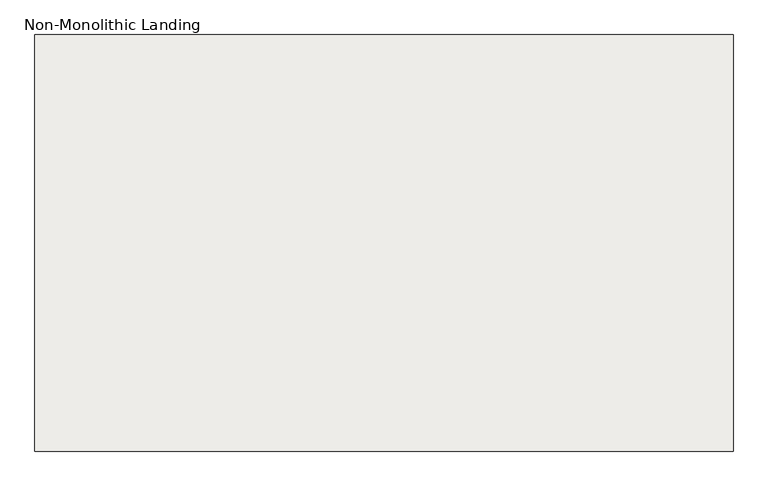
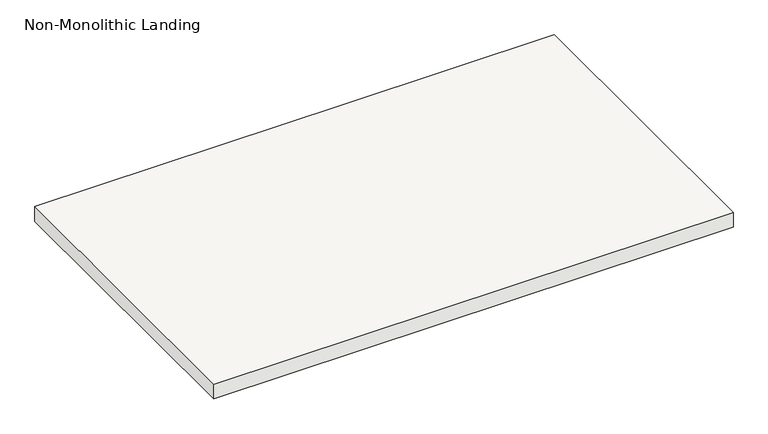
"""IFC4 building model written with IfcOpenShell, lengths in millimetres: slab geometry, Non-Monolithic Landing."""

from ifc_helpers import new_model, si_unit, frame, origin, place, context, project, spatial, polyline, outline, extrude, source, transform, mapped, element, save


def non_monolithic_landing_c5efd80b(model_context):
    return source(origin(), model_context, "Body", "SweptSolid", [
        extrude(outline(polyline([(-12626.101437, -2240.1378151), (-11950.3449834, -2240.1378151), (-11950.3449834, -3240.1378151), (-13626.101437, -3240.1378151), (-13626.101437, -2240.1378151), (-12626.101437, -2240.1378151)])), frame((0.0, 0.0, 1859.0909091), z_axis=(0.0, 0.0, 1.0), x_axis=(1.0, 0.0, 0.0)), (0.0, 0.0, 1.0), 50.0),
    ])


if __name__ == "__main__":
    model = new_model("IFC4")
    model_context = context("Model", 3, world=origin())
    ifc_project = project(units=[si_unit("LENGTHUNIT", "METRE", prefix="MILLI")], contexts=[model_context])
    site = spatial("IfcSite", under=ifc_project)
    building = spatial("IfcBuilding", under=site)
    placement = place(None, origin())
    non_monolithic_landing_shape = non_monolithic_landing_c5efd80b(model_context)
    element("IfcSlab", 1, ObjectType="Non-Monolithic Landing", at=placement, inside=building, context=model_context, shape_type="MappedRepresentation", body=[
        mapped(non_monolithic_landing_shape, transform((0.0, 0.0, 0.0), x_axis=(1.0, 0.0, 0.0), y_axis=(0.0, 1.0, 0.0), z_axis=(0.0, 0.0, 1.0))),
    ])
    save(model, "model.ifc")
